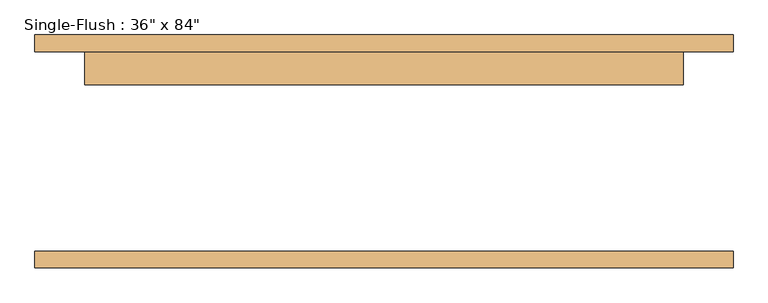
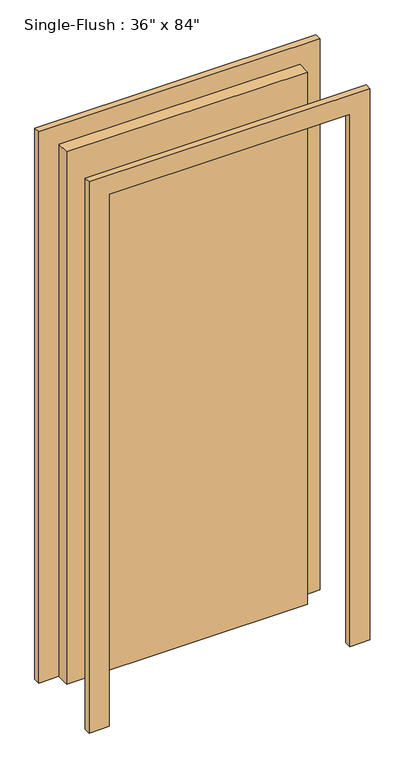
"""IFC4 building model written with IfcOpenShell, lengths in millimetres: door geometry."""

import ifcopenshell
import ifcopenshell.guid

model = None  # the IFC model being written
_history = None  # IfcOwnerHistory: only IFC2X3 demands one
_inside = {}  # id of a spatial element -> (the spatial element, [elements in it])
_under = {}  # id of a project, library or spatial element -> (it, [spatial elements below it])
_declared = {}  # id of a project -> (the project, [libraries it declares])
_typed = {}  # id of a type object -> (the type object, [elements of that type])
_made_of = {}  # id of a material, layer set ... -> (it, [elements and type objects made of it])


def new_model(schema):
    """Start an empty IFC model of exactly this schema.

    Asked for "IFC4X3", IfcOpenShell would pick the latest addendum, in which some entities
    have other attributes; the version numbers below select the first issue.
    IFC2X3 requires an IfcOwnerHistory on every rooted entity: one is made here for all.
    """
    global model, _history
    if schema == "IFC4X3":
        model = ifcopenshell.file(schema_version=(4, 3, 0, 0))
    else:
        model = ifcopenshell.file(schema=schema)
    _inside.clear()
    _under.clear()
    _declared.clear()
    _typed.clear()
    _made_of.clear()
    _history = None
    if model.schema == "IFC2X3":
        org = make("IfcOrganization", Name="unknown")
        user = make(
            "IfcPersonAndOrganization",
            ThePerson=make("IfcPerson", FamilyName="unknown"),
            TheOrganization=org,
        )
        app = make(
            "IfcApplication",
            ApplicationDeveloper=org,
            Version="unknown",
            ApplicationFullName="unknown",
            ApplicationIdentifier="unknown",
        )
        _history = make(
            "IfcOwnerHistory",
            OwningUser=user,
            OwningApplication=app,
            ChangeAction="ADDED",
            CreationDate=0,
        )
    return model


def make(cls, **values):
    """One entity of the class cls with the attributes given. An attribute that is None is left unset."""
    return model.create_entity(
        cls, **{name: value for name, value in values.items() if value is not None}
    )


def rooted(cls, **values):
    """An entity with a GlobalId (a new one), such as an element, a storey or a relation."""
    return make(cls, GlobalId=ifcopenshell.guid.new(), OwnerHistory=_history, **values)


def si_unit(unit_type, name, prefix=None):
    """IfcSIUnit, for example si_unit("LENGTHUNIT", "METRE", prefix="MILLI")."""
    return make("IfcSIUnit", UnitType=unit_type, Prefix=prefix, Name=name)


def assignment(units):
    """IfcUnitAssignment: the units of a project."""
    return None if units is None else make("IfcUnitAssignment", Units=units)


def point(xyz):
    """IfcCartesianPoint."""
    return None if xyz is None else make("IfcCartesianPoint", Coordinates=xyz)


def direction(xyz):
    """IfcDirection."""
    return None if xyz is None else make("IfcDirection", DirectionRatios=xyz)


def frame(location, z_axis=None, x_axis=None):
    """IfcAxis2Placement3D, a coordinate frame: its origin and axes. An axis left out is left unset."""
    return make(
        "IfcAxis2Placement3D",
        Location=point(location),
        Axis=direction(z_axis),
        RefDirection=direction(x_axis),
    )


def origin():
    """The frame at (0, 0, 0) with its axes left unset."""
    return frame((0.0, 0.0, 0.0))


def origin_with_axes():
    """The frame at (0, 0, 0) with the z axis (0, 0, 1) and the x axis (1, 0, 0) written out."""
    return frame((0.0, 0.0, 0.0), z_axis=(0.0, 0.0, 1.0), x_axis=(1.0, 0.0, 0.0))


def place(relative_to, where):
    """IfcLocalPlacement: puts the frame where relative to a parent placement (None: the world)."""
    return make(
        "IfcLocalPlacement", PlacementRelTo=relative_to, RelativePlacement=where
    )


def context(
    kind, dimensions, precision=None, world=None, true_north=None, identifier=None
):
    """IfcGeometricRepresentationContext, for example the 3D "Model" context."""
    return make(
        "IfcGeometricRepresentationContext",
        ContextIdentifier=identifier,
        ContextType=kind,
        CoordinateSpaceDimension=dimensions,
        Precision=precision,
        WorldCoordinateSystem=world,
        TrueNorth=true_north,
    )


def project(units=None, contexts=None):
    """IfcProject with its units and contexts."""
    return rooted(
        "IfcProject",
        Name="project",
        RepresentationContexts=contexts,
        UnitsInContext=assignment(units),
    )


def spatial(cls, under=None, at=None, **own):
    """A site, building, storey or space (cls), placed at a placement, below another one or the project."""
    s = rooted(cls, ObjectPlacement=at, **own)
    if under is not None:
        _under.setdefault(under.id(), (under, []))[1].append(s)
    return s


def polyline(points):
    """IfcPolyline through the points."""
    return make("IfcPolyline", Points=[point(p) for p in points])


def outline(outer, holes=None, kind="AREA"):
    """IfcArbitraryClosedProfileDef: a profile drawn as a closed curve; with holes, ...WithVoids."""
    if holes is None:
        return make("IfcArbitraryClosedProfileDef", ProfileType=kind, OuterCurve=outer)
    return make(
        "IfcArbitraryProfileDefWithVoids",
        ProfileType=kind,
        OuterCurve=outer,
        InnerCurves=holes,
    )


def extrude(swept, where, along, depth):
    """IfcExtrudedAreaSolid: the profile swept, set in the frame where, extruded along a direction by depth."""
    return make(
        "IfcExtrudedAreaSolid",
        SweptArea=swept,
        Position=where,
        ExtrudedDirection=direction(along),
        Depth=depth,
    )


def shape(context_of_items, identifier, shape_type, items):
    """IfcShapeRepresentation: the items that make up one representation, for example the "Body"."""
    return make(
        "IfcShapeRepresentation",
        ContextOfItems=context_of_items,
        RepresentationIdentifier=identifier,
        RepresentationType=shape_type,
        Items=items,
    )


def source(mapping_origin, context_of_items, identifier, shape_type, items):
    """IfcRepresentationMap: a shape defined once, which mapped items show again and again."""
    return make(
        "IfcRepresentationMap",
        MappingOrigin=mapping_origin,
        MappedRepresentation=shape(context_of_items, identifier, shape_type, items),
    )


def transform(
    local_origin,
    x_axis=None,
    y_axis=None,
    z_axis=None,
    scale=None,
    scale2=None,
    scale3=None,
    uniform=True,
):
    """IfcCartesianTransformationOperator3D, or its non-uniform kind. x_axis, y_axis, z_axis: its Axis1, 2, 3."""
    if uniform:
        return make(
            "IfcCartesianTransformationOperator3D",
            Axis1=direction(x_axis),
            Axis2=direction(y_axis),
            LocalOrigin=point(local_origin),
            Scale=scale,
            Axis3=direction(z_axis),
        )
    return make(
        "IfcCartesianTransformationOperator3DnonUniform",
        Axis1=direction(x_axis),
        Axis2=direction(y_axis),
        LocalOrigin=point(local_origin),
        Scale=scale,
        Axis3=direction(z_axis),
        Scale2=scale2,
        Scale3=scale3,
    )


def mapped(mapping_source, mapping_target):
    """IfcMappedItem: shows the shape of a source again, moved by a transform."""
    return make(
        "IfcMappedItem", MappingSource=mapping_source, MappingTarget=mapping_target
    )


def made_of(thing, what):
    """Note that an element or type object is made of a material, layer set ...; save() writes the relation."""
    if what is not None:
        _made_of.setdefault(what.id(), (what, []))[1].append(thing)
    return thing


def element(
    cls,
    number,
    at=None,
    inside=None,
    cuts=None,
    type_object=None,
    material=None,
    context=None,
    identifier="Body",
    shape_type=None,
    held_by="IfcProductDefinitionShape",
    body=None,
    shapes=None,
    **own,
):
    """One element of the class cls, such as IfcWall. Its Tag is "e" and its number.

    at: its placement. inside: the storey or other place that contains it. cuts: it is an
    opening in that element (IfcRelVoidsElement). A single representation is given by context,
    identifier, shape_type and body (its items); several are given by shapes. held_by: the class
    of the entity that holds the representations. save() writes the other relations.
    """
    e = rooted(cls, Tag="e%d" % number, ObjectPlacement=at, **own)
    if body is not None:
        shapes = [shape(context, identifier, shape_type, body)]
    if shapes is not None:
        e.Representation = make(held_by, Representations=shapes)
    if inside is not None:
        _inside.setdefault(inside.id(), (inside, []))[1].append(e)
    if cuts is not None:
        rooted(
            "IfcRelVoidsElement", RelatingBuildingElement=cuts, RelatedOpeningElement=e
        )
    if type_object is not None:
        _typed.setdefault(type_object.id(), (type_object, []))[1].append(e)
    return made_of(e, material)


def aggregate(whole, parts):
    """IfcRelAggregates: a whole, such as a stair, and the parts it consists of."""
    return rooted("IfcRelAggregates", RelatingObject=whole, RelatedObjects=parts)


def save(model, path):
    """Write the relations noted so far, then the file.

    IfcRelAggregates (storeys below a building ...), IfcRelContainedInSpatialStructure (elements
    in a storey), IfcRelDefinesByType, IfcRelAssociatesMaterial and IfcRelDeclares: one each for
    every whole, place, type object, material and project.
    """
    for whole, parts in _under.values():
        aggregate(whole, parts)
    for where, things in _inside.values():
        rooted(
            "IfcRelContainedInSpatialStructure",
            RelatedElements=things,
            RelatingStructure=where,
        )
    for kind, things in _typed.values():
        rooted("IfcRelDefinesByType", RelatedObjects=things, RelatingType=kind)
    for what, things in _made_of.values():
        rooted("IfcRelAssociatesMaterial", RelatedObjects=things, RelatingMaterial=what)
    for by, libraries in _declared.values():
        rooted("IfcRelDeclares", RelatingContext=by, RelatedDefinitions=libraries)
    model.write(path)


def door_03272193(model_context):
    return source(origin(), model_context, "Body", "SweptSolid", [
        extrude(outline(polyline([(2209.8, -533.4), (0.0, -533.4), (0.0, -457.2), (2133.6, -457.2), (2133.6, 457.2), (0.0, 457.2), (0.0, 533.4), (2209.8, 533.4), (2209.8, -533.4)])), frame((0.0, 152.4, 0.0), z_axis=(0.0, 1.0, 0.0), x_axis=(0.0, 0.0, 1.0)), (0.0, 0.0, 1.0), 25.4),
        extrude(outline(polyline([(2209.8, 533.4), (2209.8, -533.4), (0.0, -533.4), (0.0, -457.2), (2133.6, -457.2), (2133.6, 457.2), (0.0, 457.2), (0.0, 533.4), (2209.8, 533.4)])), frame((0.0, -177.8, 0.0), z_axis=(0.0, 1.0, 0.0), x_axis=(0.0, 0.0, 1.0)), (0.0, 0.0, 1.0), 25.4),
        extrude(outline(polyline([(457.2, 101.6), (-457.2, 101.6), (-457.2, 152.4), (457.2, 152.4), (457.2, 101.6)])), origin_with_axes(), (0.0, 0.0, 1.0), 2133.6),
    ])


if __name__ == "__main__":
    model = new_model("IFC4")
    model_context = context("Model", 3, world=origin())
    ifc_project = project(units=[si_unit("LENGTHUNIT", "METRE", prefix="MILLI")], contexts=[model_context])
    site = spatial("IfcSite", under=ifc_project)
    building = spatial("IfcBuilding", under=site)
    placement = place(None, origin())
    door_shape = door_03272193(model_context)
    element("IfcDoor", 1, ObjectType="Single-Flush : 36\" x 84\"", at=placement, inside=building, context=model_context, shape_type="MappedRepresentation", body=[
        mapped(door_shape, transform((0.0, 0.0, 0.0), x_axis=(1.0, 0.0, 0.0), y_axis=(0.0, 1.0, 0.0), z_axis=(0.0, 0.0, 1.0))),
    ])
    save(model, "model.ifc")

# Revit data of these elements
# Type "Single-Flush : 36\" x 84\""
#   Type Mark = "1"
#   Construction Type Id = "MDOOR"
#   Assembly Code = "C1020"
#   Analytic Construction = "Metal"
#   Thickness = 0' - 2"
#   Heat Transfer Coefficient (U) = 0.651978 BTU/(h·ft²·°F)
#   Height = 7' - 0"
#   Trim Projection Ext = 0' - 1"
#   Trim Projection Int = 0' - 1"
#   Trim Width = 0' - 3"
#   Width = 3' - 0"
#   Define Thermal Properties by = 1
#   Define Thermal Properties by = 1
#   Door Material = Door - Panel
#   Frame Material = Door - Frame
#   Visual Light Transmittance = 0
#   Solar Heat Gain Coefficient = 0
#   Function = (empty or 0)
#   Wall Closure = (empty or 0)
# Element 1 (IfcDoor, "Single-Flush : 36\" x 84\"")
#   Materials on its faces: "Door - Frame", "Door - Panel"
# Materials
#   "Door - Panel": class "Wood", colour RGB 210 159 95, transparency 0, Cost = 0
#   "Door - Frame": class "Miscellaneous", colour RGB 118 70 51, transparency 0, Cost = 0
